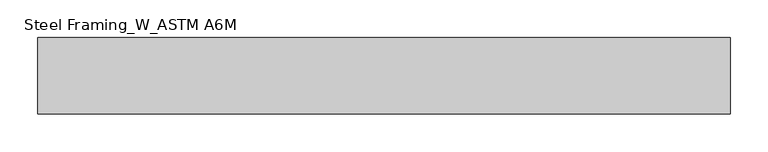
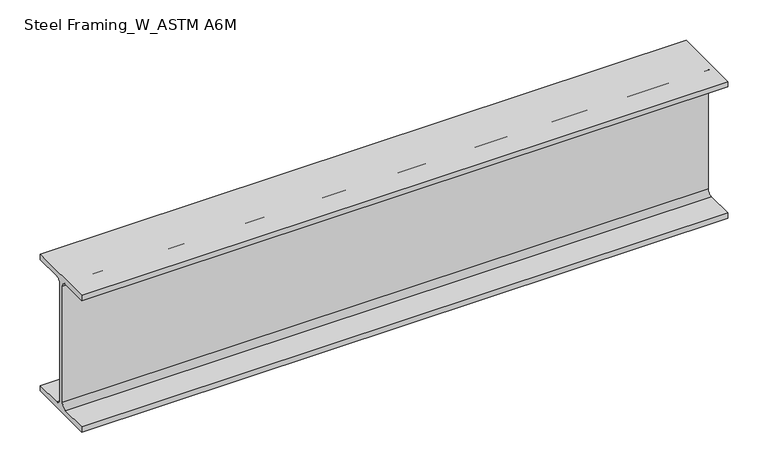
"""IFC4 building model written with IfcOpenShell, lengths in millimetres: beam geometry, Steel Framing_W_ASTM A6M : H_SB_AR_S02_W200x22.5_J1."""

from ifc_helpers import new_model, si_unit, point, frame, frame_2d, origin, place, context, project, spatial, polyline, circle_curve, trimmed, segment, composite_curve, outline, extrude, source, transform, mapped, element, save


def steel_framing_w_astm_a6m_c1a3e6cc(model_context):
    return source(origin(), model_context, "Body", "SweptSolid", [
        extrude(outline(composite_curve([segment(polyline([(51.0, -95.0), (51.0, -103.0), (-51.0, -103.0), (-51.0, -95.0), (-10.71, -95.0)]), True, "CONTINUOUS"), segment(trimmed(circle_curve(frame_2d((-10.71, -87.4)), 7.6), [point((-10.71, -95.0))], [point((-3.11, -87.4))], True, "CARTESIAN"), True, "CONTINUOUS"), segment(polyline([(-3.11, -87.4), (-3.11, 87.4)]), True, "CONTINUOUS"), segment(trimmed(circle_curve(frame_2d((-10.71, 87.4)), 7.6), [point((-3.11, 87.4))], [point((-10.71, 95.0))], True, "CARTESIAN"), True, "CONTINUOUS"), segment(polyline([(-10.71, 95.0), (-51.0, 95.0), (-51.0, 103.0), (51.0, 103.0), (51.0, 95.0), (10.71, 95.0)]), True, "CONTINUOUS"), segment(trimmed(circle_curve(frame_2d((10.71, 87.4)), 7.6), [point((10.71, 95.0))], [point((3.11, 87.4))], True, "CARTESIAN"), True, "CONTINUOUS"), segment(polyline([(3.11, 87.4), (3.11, -87.4)]), True, "CONTINUOUS"), segment(trimmed(circle_curve(frame_2d((10.71, -87.4)), 7.6), [point((3.11, -87.4))], [point((10.71, -95.0))], True, "CARTESIAN"), True, "CONTINUOUS"), segment(polyline([(10.71, -95.0), (51.0, -95.0)]), True, "CONTINUOUS")], self_intersect=False)), frame((-460.3, 0.0, 0.0), z_axis=(1.0, 0.0, 0.0), x_axis=(0.0, 1.0, 0.0)), (0.0, 0.0, 1.0), 920.6),
    ])


if __name__ == "__main__":
    model = new_model("IFC4")
    model_context = context("Model", 3, world=origin())
    ifc_project = project(units=[si_unit("LENGTHUNIT", "METRE", prefix="MILLI")], contexts=[model_context])
    site = spatial("IfcSite", under=ifc_project)
    building = spatial("IfcBuilding", under=site)
    placement = place(None, origin())
    steel_framing_w_astm_a6m_shape = steel_framing_w_astm_a6m_c1a3e6cc(model_context)
    element("IfcBeam", 1, ObjectType="Steel Framing_W_ASTM A6M : H_SB_AR_S02_W200x22.5_J1", at=placement, inside=building, context=model_context, shape_type="MappedRepresentation", body=[
        mapped(steel_framing_w_astm_a6m_shape, transform((0.0, 0.0, 0.0), x_axis=(1.0, 0.0, 0.0), y_axis=(0.0, 1.0, 0.0), z_axis=(0.0, 0.0, 1.0))),
    ])
    save(model, "model.ifc")

# Revit data of these elements
# Type "Steel Framing_W_ASTM A6M : H_SB_AR_S02_W200x22.5_J1"
#   Section Name Key = "W8x15"
#   Width = 10.2 cm
#   Web Thickness = 0.622 cm
#   Web Fillet = 0.76 cm
#   Warping Constant = 13900.0 cm⁶
#   Torsional Moment of Inertia = 5.70 cm⁴
#   Section Area = 28.6 cm²
#   Plastic Modulus weak axis = 43.8 cm³
#   Plastic Modulus strong axis = 223.0 cm³
#   Perimeter = 0.795 m²/m
#   Nominal Weight = 22.50 kgf/m
#   Moment of Inertia weak axis = 142.00 cm⁴
#   Moment of Inertia strong axis = 2000.00 cm⁴
#   Height = 20.6 cm
#   Flange Thickness = 0.8 cm
#   Elastic Modulus weak axis = 27.9 cm³
#   Elastic Modulus strong axis = 193.0 cm³
#   Centroid Vertical = 10.3 cm
#   Centroid Horizontal = 5.1 cm
#   Length [instance default] = 1500 mm
#   Structural Material [instance default] = Steel, 45-345
#   Bolt Spacing = 0
#   Assembly Code = ""
# Element 1 (IfcBeam, "Steel Framing_W_ASTM A6M : H_SB_AR_S02_W200x22.5_J1")
#   Materials on its faces: "Steel, 45-345"
# Materials
#   "Steel, 45-345": class "Metal", colour RGB 189 187 185, transparency 0, Description = "Steel 345 MPa", Cost = 0
